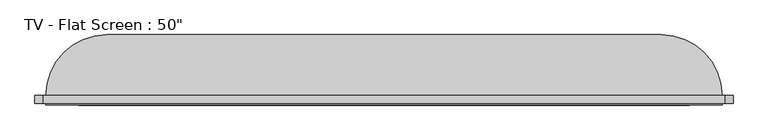
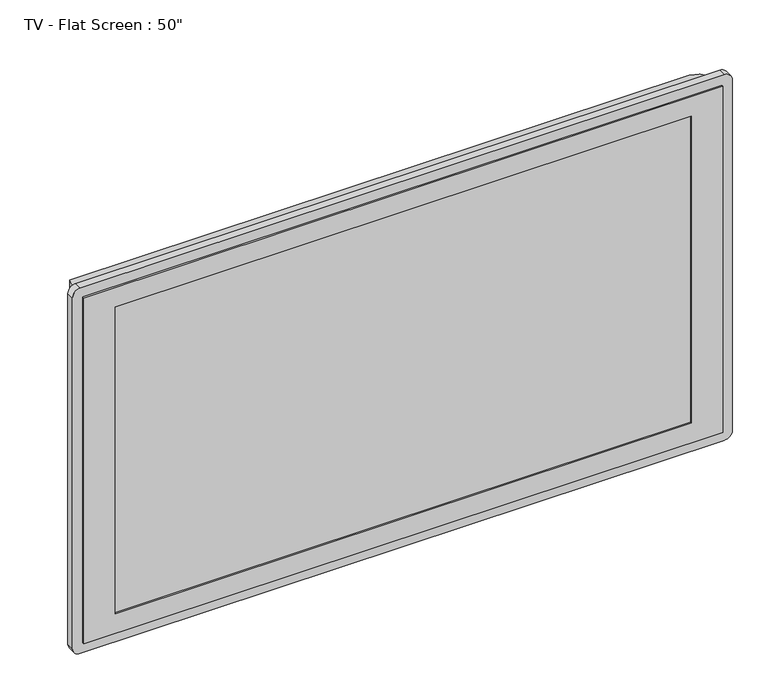
"""IFC4 building model written with IfcOpenShell, lengths in millimetres: furniture geometry."""

from ifc_helpers import new_model, si_unit, point, frame, frame_2d, origin, place, context, project, spatial, polyline, circle_curve, ellipse_curve, trimmed, segment, composite_curve, outline, extrude, faceted_brep, source, transform, mapped, element, save
from ifc_brep_helpers import plane_surface, cylinder_surface, advanced_brep


def furniture_dedffa24(model_context):
    return source(origin(), model_context, "Body", "SolidModel", [
        faceted_brep([(609.4937454, -69.4613764, 782.6751733), (-617.3827737, -69.4613764, 782.6751733), (-617.3827737, -69.4613764, 80.0), (609.4937454, -69.4613764, 80.0), (-557.3827737, -69.4613764, 742.6751733), (549.4937454, -69.4613764, 742.6751733), (549.4937454, -69.4613764, 120.0), (-557.3827737, -69.4613764, 120.0), (609.4937454, -51.4613764, 782.6751733), (609.4937454, -51.4613764, 80.0), (-617.3827737, -51.4613764, 80.0), (-617.3827737, -51.4613764, 782.6751733), (-557.3827737, -66.4613764, 742.6751733), (-557.3827737, -66.4613764, 120.0), (549.4937454, -66.4613764, 120.0), (549.4937454, -66.4613764, 742.6751733)], [[[0, 1, 2, 3], [4, 5, 6, 7]], [[8, 9, 10, 11]], [[1, 0, 8, 11]], [[2, 1, 11, 10]], [[3, 2, 10, 9]], [[0, 3, 9, 8]], [[12, 13, 14, 15]], [[12, 15, 5, 4]], [[15, 14, 6, 5]], [[14, 13, 7, 6]], [[13, 12, 4, 7]]]),
        extrude(outline(composite_curve([segment(polyline([(802.6751733, 614.4937454), (802.6751733, -622.3827737)]), True, "CONTINUOUS"), segment(trimmed(circle_curve(frame_2d((787.6751733, -622.3827737)), 15.0), [point((802.6751733, -622.3827737))], [point((787.6751733, -637.3827737))], False, "CARTESIAN"), True, "CONTINUOUS"), segment(polyline([(787.6751733, -637.3827737), (75.0, -637.3827737)]), True, "CONTINUOUS"), segment(trimmed(circle_curve(frame_2d((75.0, -622.3827737)), 15.0), [point((75.0, -637.3827737))], [point((60.0, -622.3827737))], False, "CARTESIAN"), True, "CONTINUOUS"), segment(polyline([(60.0, -622.3827737), (60.0, 614.4937454)]), True, "CONTINUOUS"), segment(trimmed(circle_curve(frame_2d((75.0, 614.4937454)), 15.0), [point((60.0, 614.4937454))], [point((75.0, 629.4937454))], False, "CARTESIAN"), True, "CONTINUOUS"), segment(polyline([(75.0, 629.4937454), (787.6751733, 629.4937454)]), True, "CONTINUOUS"), segment(trimmed(circle_curve(frame_2d((787.6751733, 614.4937454)), 15.0), [point((787.6751733, 629.4937454))], [point((802.6751733, 614.4937454))], False, "CARTESIAN"), True, "CONTINUOUS")], self_intersect=False), holes=[polyline([(782.6751733, 609.4937454), (80.0, 609.4937454), (80.0, -617.3827737), (782.6751733, -617.3827737), (782.6751733, 609.4937454)])]), frame((0.0, -66.4613764, 0.0), z_axis=(0.0, 1.0, 0.0), x_axis=(0.0, 0.0, 1.0)), (0.0, 0.0, 1.0), 15.0),
        advanced_brep(
        [(-617.3827737, -51.4613764, 80.0), (609.4937454, -51.4613764, 80.0), (609.4937454, -51.4613764, 782.6751733), (-617.3827737, -51.4613764, 782.6751733), (499.4937454, 58.5386236, 80.0), (-507.3827737, 58.5386236, 80.0), (-507.3827737, 58.5386236, 672.6751733), (499.4937454, 58.5386236, 672.6751733)],
        [
            (0, 1),
            (1, 2),
            (2, 3),
            (3, 0),
            (4, 5),
            (5, 6),
            (6, 7),
            (7, 4),
            (0, 5, circle_curve(frame((-507.3827737, -51.4613764, 80.0), z_axis=(0.0, 0.0, -1.0), x_axis=(-1.0, 0.0, 0.0)), 110.0)),
            (4, 1, circle_curve(frame((499.4937454, -51.4613764, 80.0), z_axis=(0.0, 0.0, -1.0), x_axis=(1.0, 0.0, 0.0)), 110.0)),
            (7, 2, ellipse_curve(frame((499.4937454, -51.4613764, 672.6751733), z_axis=(0.7071067811865475, 0.0, -0.7071067811865475), x_axis=(0.7071067811865474, 0.0, 0.7071067811865476)), 155.5634919, 110.0)),
            (6, 3, ellipse_curve(frame((-507.3827737, -51.4613764, 672.6751733), z_axis=(0.7071067811865475, 0.0, 0.7071067811865475), x_axis=(-0.7071067811865476, 0.0, 0.7071067811865474)), 155.5634919, 110.0)),
        ],
        [
            plane_surface(frame((-617.3827737, -51.4613764, 782.6751733), z_axis=(0.0, -1.0, 0.0), x_axis=(-1.0, 0.0, 0.0))),
            plane_surface(frame((-617.3827737, 58.5386236, 782.6751733), z_axis=(0.0, 1.0, 0.0), x_axis=(1.0, 0.0, 0.0))),
            plane_surface(frame((-617.3827737, -51.4613764, 80.0), z_axis=(0.0, 0.0, -1.0), x_axis=(0.0, 1.0, 0.0))),
            cylinder_surface(frame((499.4937454, -51.4613764, 80.0), z_axis=(0.0, 0.0, 1.0), x_axis=(1.0, 0.0, 0.0)), 110.0),
            cylinder_surface(frame((609.4937454, -51.4613764, 672.6751733), z_axis=(-1.0, 0.0, 0.0), x_axis=(0.0, 0.0, 1.0)), 110.0),
            cylinder_surface(frame((-507.3827737, -51.4613764, 782.6751733), z_axis=(0.0, 0.0, -1.0), x_axis=(-1.0, 0.0, 0.0)), 110.0),
        ],
        [
            (0, [[1, 2, 3, 4]]),
            (1, [[5, 6, 7, 8]]),
            (2, [[-1, 9, -5, 10]]),
            (3, [[11, -2, -10, -8]]),
            (4, [[-11, -7, 12, -3]]),
            (5, [[-12, -6, -9, -4]]),
        ],
    ),
    ])


if __name__ == "__main__":
    model = new_model("IFC4")
    model_context = context("Model", 3, world=origin())
    ifc_project = project(units=[si_unit("LENGTHUNIT", "METRE", prefix="MILLI")], contexts=[model_context])
    site = spatial("IfcSite", under=ifc_project)
    building = spatial("IfcBuilding", under=site)
    placement = place(None, origin())
    furniture_shape = furniture_dedffa24(model_context)
    element("IfcFurniture", 1, ObjectType="TV - Flat Screen : 50\"", at=placement, inside=building, context=model_context, shape_type="MappedRepresentation", body=[
        mapped(furniture_shape, transform((0.0, 0.0, 0.0), x_axis=(1.0, 0.0, 0.0), y_axis=(0.0, 1.0, 0.0), z_axis=(0.0, 0.0, 1.0))),
    ])
    save(model, "model.ifc")

# Revit data of these elements
# Type "TV - Flat Screen : 50\""
#   Model = "TV50"
#   Manufacturer = "Corporate Concepts"
#   Type Mark = "TV-1"
#   Cost = 450
#   SinAng = 0' - 0.0193"
#   L = 3' - 7.57782"
#   H = 2' - 0.51477"
#   Thickness = 0' - 4.33071"
#   Diagonal = 4' - 2"
#   CosAng = 0' - 0.03431"
#   Stand [instance default] = yes
#   Default Elevation = 0
# Element 1 (IfcFurniture, "TV - Flat Screen : 50\"")
#   Stand = no
#   Materials on its faces: "TV - Black", "TV - Glass", "TV - Screen"
# Materials
#   "TV - Black": class "Miscellaneous", colour RGB 49 49 49, transparency 0
#   "TV - Glass": class "Miscellaneous", colour RGB 157 157 157, transparency 0.9
#   "TV - Screen": class "Miscellaneous", colour RGB 0 0 0, transparency 0
